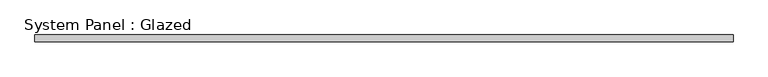
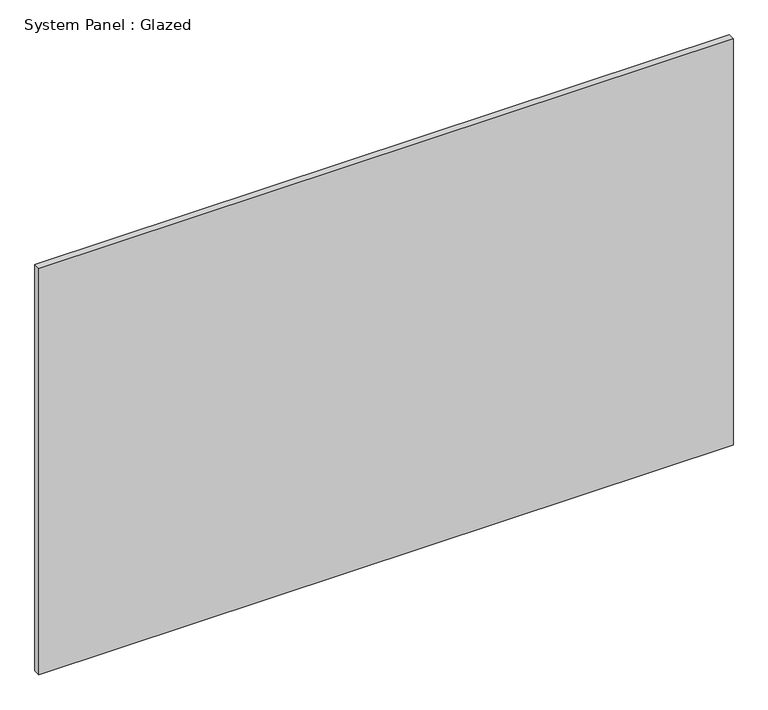
"""IFC4 building model written with IfcOpenShell, lengths in millimetres: plate geometry, System Panel : Glazed."""

from ifc_helpers import new_model, si_unit, origin, origin_with_axes, place, context, project, spatial, polyline, outline, extrude, source, transform, mapped, element, save


def system_panel_glazed_5afca271(model_context):
    return source(origin(), model_context, "Body", "SweptSolid", [
        extrude(outline(polyline([(1232.875, 24.5), (-1232.875, 24.5), (-1232.875, 49.5), (1232.875, 49.5), (1232.875, 24.5)])), origin_with_axes(), (0.0, 0.0, 1.0), 1526.020449),
    ])


if __name__ == "__main__":
    model = new_model("IFC4")
    model_context = context("Model", 3, world=origin())
    ifc_project = project(units=[si_unit("LENGTHUNIT", "METRE", prefix="MILLI")], contexts=[model_context])
    site = spatial("IfcSite", under=ifc_project)
    building = spatial("IfcBuilding", under=site)
    placement = place(None, origin())
    system_panel_glazed_shape = system_panel_glazed_5afca271(model_context)
    element("IfcPlate", 1, ObjectType="System Panel : Glazed", at=placement, inside=building, context=model_context, shape_type="MappedRepresentation", body=[
        mapped(system_panel_glazed_shape, transform((0.0, 0.0, 0.0), x_axis=(1.0, 0.0, 0.0), y_axis=(0.0, 1.0, 0.0), z_axis=(0.0, 0.0, 1.0))),
    ])
    save(model, "model.ifc")

# Revit data of these elements
# Type "System Panel : Glazed"
#   Keynote = "H11"
#   Construction Type Id = "GSP4R"
#   Analytic Construction = "1/8 in Pilkington single glazing"
#   Visual Light Transmittance = 0.9
#   Solar Heat Gain Coefficient = 0.86
#   Heat Transfer Coefficient (U) = 6.7069 W/(m²·K)
#   Define Thermal Properties by = 1
# Element 1 (IfcPlate, "System Panel : Glazed")
#   Materials on its faces: "Glass"
# Materials
#   "Glass": class "Glass", colour RGB 0 128 192, transparency 0.9, Description = "Soda Lime Glass", Cost = 0
